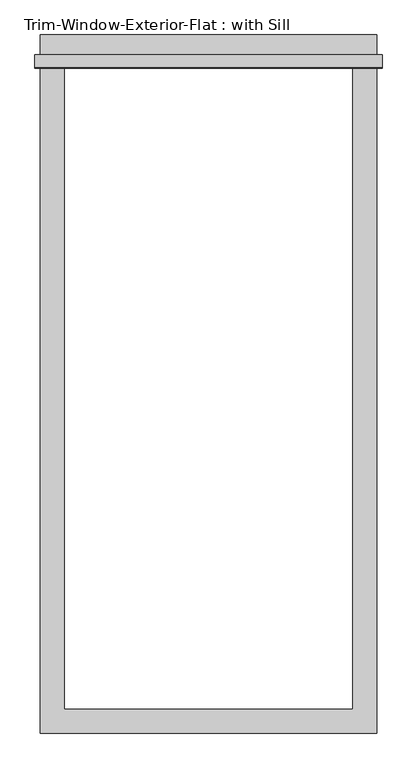
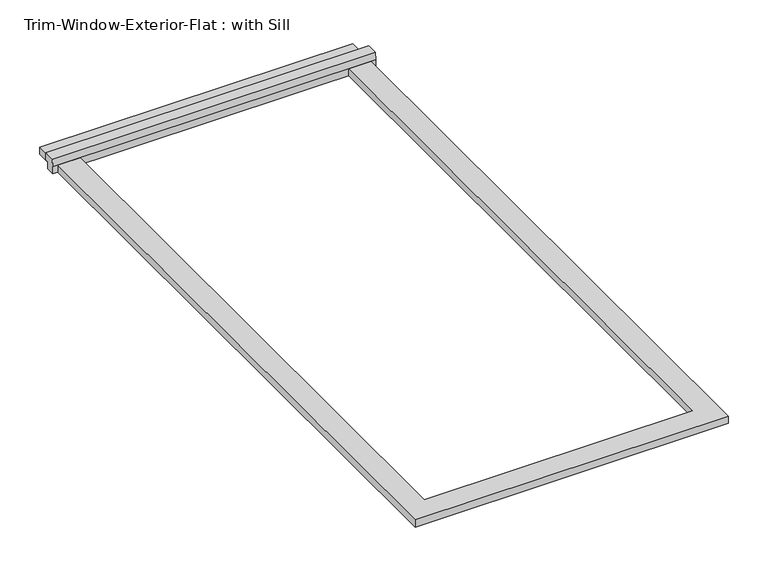
"""IFC4 building model written with IfcOpenShell, lengths in millimetres: proxy geometry, Trim-Window-Exterior-Flat : with Sill."""

from ifc_helpers import new_model, si_unit, frame, origin, origin_with_axes, place, context, project, spatial, polyline, outline, extrude, source, transform, mapped, element, save


def trim_window_exterior_flat_with_sill_504c3d8a(model_context):
    return source(origin(), model_context, "Body", "SweptSolid", [
        extrude(outline(polyline([(400.05, 1546.1823709), (-400.05, 1546.1823709), (-400.05, 1603.3323709), (400.05, 1603.3323709), (400.05, 1546.1823709)])), origin_with_axes(), (0.0, 0.0, 1.0), 19.05),
        extrude(outline(polyline([(1555.75, 38.1), (1555.75, 19.05), (1546.1823709, 19.05), (1546.1823709, 0.0), (1524.0, 0.0), (1524.0, 19.05), (1526.4580645, 38.1), (1555.75, 38.1)])), frame((-412.75, 0.0, 0.0), z_axis=(1.0, 0.0, 0.0), x_axis=(0.0, 1.0, 0.0)), (0.0, 0.0, 1.0), 825.5),
        extrude(outline(polyline([(-400.05, -57.15), (-400.05, 1524.0), (-342.9, 1524.0), (-342.9, 0.0), (342.9, 0.0), (342.9, 1524.0), (400.05, 1524.0), (400.05, -57.15), (-400.05, -57.15)])), origin_with_axes(), (0.0, 0.0, 1.0), 19.05),
    ])


if __name__ == "__main__":
    model = new_model("IFC4")
    model_context = context("Model", 3, world=origin())
    ifc_project = project(units=[si_unit("LENGTHUNIT", "METRE", prefix="MILLI")], contexts=[model_context])
    site = spatial("IfcSite", under=ifc_project)
    building = spatial("IfcBuilding", under=site)
    placement = place(None, origin())
    trim_window_exterior_flat_with_sill_shape = trim_window_exterior_flat_with_sill_504c3d8a(model_context)
    element("IfcBuildingElementProxy", 1, Name="Trim-Window-Exterior-Flat : with Sill", ObjectType="Trim-Window-Exterior-Flat : with Sill", at=placement, inside=building, context=model_context, shape_type="MappedRepresentation", body=[
        mapped(trim_window_exterior_flat_with_sill_shape, transform((0.0, 0.0, 0.0), x_axis=(1.0, 0.0, 0.0), y_axis=(0.0, 1.0, 0.0), z_axis=(0.0, 0.0, 1.0))),
    ])
    save(model, "model.ifc")

# Revit data of these elements
# Type "Trim-Window-Exterior-Flat : with Sill"
#   Trim Width = 0' - 2 1/4"
#   Trim Thickness_Picture Frame = 0' - 1 1/4"
#   Trim Thickness_with Sill = 0' - 0 3/4"
#   Sill Thickness = 0' - 1 1/4"
#   Opening Width [instance default] = 2' - 0"
#   Opening Height [instance default] = 3' - 0"
#   Default Elevation = 4' - 0"
#   Sill = yes
#   Picture Frame = no
#   Trim Material [instance default] = none
# Element 1 (IfcBuildingElementProxy, "Trim-Window-Exterior-Flat : with Sill")
#   Opening Width = 2' - 3"
#   Opening Height = 5' - 0"
#   Trim Material = Clad - White
#   Materials on its faces: "Clad - White"
# Materials
#   "Clad - White": class "Wood", colour RGB 242 242 238, transparency 0, Cost = 0
